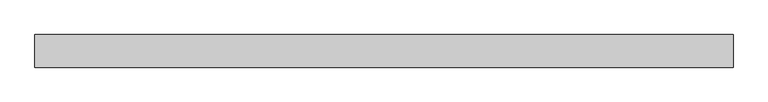
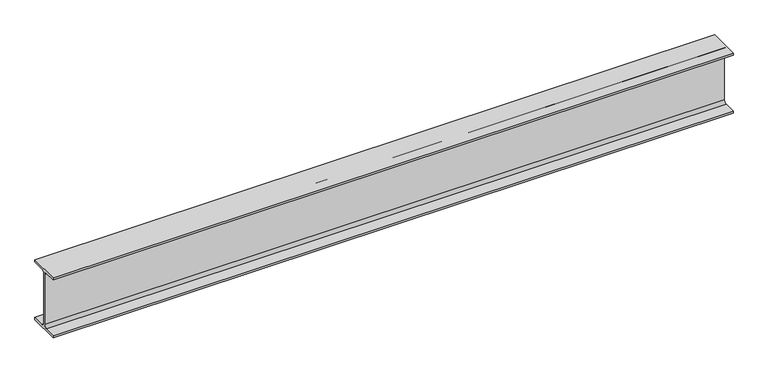
"""IFC4 building model written with IfcOpenShell, lengths in millimetres: beam geometry, 0912_Steel Framing_H-KSD3502 : H_SB_ASB_H-250x125x6x9."""

from ifc_helpers import new_model, si_unit, point, frame, frame_2d, origin, place, context, project, spatial, polyline, circle_curve, trimmed, segment, composite_curve, outline, extrude, source, transform, mapped, element, save


def beam_af623b59(model_context):
    return source(origin(), model_context, "Body", "SweptSolid", [
        extrude(outline(composite_curve([segment(polyline([(62.5, -116.0), (62.5, -125.0), (-62.5, -125.0), (-62.5, -116.0), (-15.0, -116.0)]), True, "CONTINUOUS"), segment(trimmed(circle_curve(frame_2d((-15.0, -104.0)), 12.0), [point((-15.0, -116.0))], [point((-3.0, -104.0))], True, "CARTESIAN"), True, "CONTINUOUS"), segment(polyline([(-3.0, -104.0), (-3.0, 104.0)]), True, "CONTINUOUS"), segment(trimmed(circle_curve(frame_2d((-15.0, 104.0)), 12.0), [point((-3.0, 104.0))], [point((-15.0, 116.0))], True, "CARTESIAN"), True, "CONTINUOUS"), segment(polyline([(-15.0, 116.0), (-62.5, 116.0), (-62.5, 125.0), (62.5, 125.0), (62.5, 116.0), (15.0, 116.0)]), True, "CONTINUOUS"), segment(trimmed(circle_curve(frame_2d((15.0, 104.0)), 12.0), [point((15.0, 116.0))], [point((3.0, 104.0))], True, "CARTESIAN"), True, "CONTINUOUS"), segment(polyline([(3.0, 104.0), (3.0, -104.0)]), True, "CONTINUOUS"), segment(trimmed(circle_curve(frame_2d((15.0, -104.0)), 12.0), [point((3.0, -104.0))], [point((15.0, -116.0))], True, "CARTESIAN"), True, "CONTINUOUS"), segment(polyline([(15.0, -116.0), (62.5, -116.0)]), True, "CONTINUOUS")], self_intersect=False)), frame((-1404.8000503, 0.0, 0.0), z_axis=(1.0, 0.0, 0.0), x_axis=(0.0, 1.0, 0.0)), (0.0, 0.0, 1.0), 2674.6999215),
    ])


if __name__ == "__main__":
    model = new_model("IFC4")
    model_context = context("Model", 3, world=origin())
    ifc_project = project(units=[si_unit("LENGTHUNIT", "METRE", prefix="MILLI")], contexts=[model_context])
    site = spatial("IfcSite", under=ifc_project)
    building = spatial("IfcBuilding", under=site)
    placement = place(None, origin())
    beam_shape = beam_af623b59(model_context)
    element("IfcBeam", 1, ObjectType="0912_Steel Framing_H-KSD3502 : H_SB_ASB_H-250x125x6x9", at=placement, inside=building, context=model_context, shape_type="MappedRepresentation", body=[
        mapped(beam_shape, transform((0.0, 0.0, 0.0), x_axis=(1.0, 0.0, 0.0), y_axis=(0.0, 1.0, 0.0), z_axis=(0.0, 0.0, 1.0))),
    ])
    save(model, "model.ifc")

# Revit data of these elements
# Type "0912_Steel Framing_H-KSD3502 : H_SB_ASB_H-250x125x6x9"
#   H_WM Code_1 = "S01AA003-00001 | Main Steel Structure Fabrication Work | Shelter/Building | Light Steel - Standard (30KG/M>Weight) | Material: (   )"
#   H_WM Code_2 = "S03AA029-00001 | Main Steel Structure Erection Work | Shelter/Building | Light Steel (30KG/M>Weight) | Material: (   )"
#   H_WM Code_3 = "S01AA010-00001 | Main Steel Structure Fabrication Work | Shelter/Building | Steel Painting/Coating | for Non-Fireproofed Steel Surface, Surface Preparation, Primer, Second & Final Coat | Material: (   )"
#   H_Q'ty Cal Type Tag = "SB-Q2"
#   Width = 12.5 cm
#   Web Thickness = 0.6 cm
#   Web Fillet = 1.2 cm
#   Warping Constant = 42539.8 cm⁶
#   W = 0
#   Torsional Moment of Inertia = 7.8102 cm⁴
#   Section Area = 37.66 cm²
#   Plastic Modulus weak axis = 73.1 cm³
#   Plastic Modulus strong axis = 366.0 cm³
#   Perimeter = 0.97 m²/m
#   Nominal Weight = 29.60 kgf/m
#   Moment of Inertia weak axis = 294.00 cm⁴
#   Moment of Inertia strong axis = 4050.00 cm⁴
#   Height = 25.0 cm
#   Flange Thickness = 0.9 cm
#   Elastic Modulus weak axis = 47.0 cm³
#   Elastic Modulus strong axis = 324.0 cm³
#   Centroid Vertical = 12.5 cm
#   Centroid Horizontal = 6.25 cm
#   Ix = 40500000
#   Length [instance default] = 1.5240 m
#   Zx = 366000
#   b = 0.1250 m
#   h = 0.2500 m
#   r = 0.0120 m
#   s = 0.0060 m
#   t = 0.0090 m
#   A = 0.003766 m²
#   Structural Material [instance default] = Steel, 45-345
#   Assembly Code = ""
# Element 1 (IfcBeam, "0912_Steel Framing_H-KSD3502 : H_SB_ASB_H-250x125x6x9")
#   Structural Material = none
# Materials
#   "Steel, 45-345": class "Metal", colour RGB 189 187 185, transparency 0, Description = "Steel 345 MPa", Cost = 0
